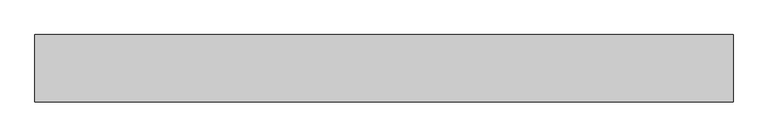
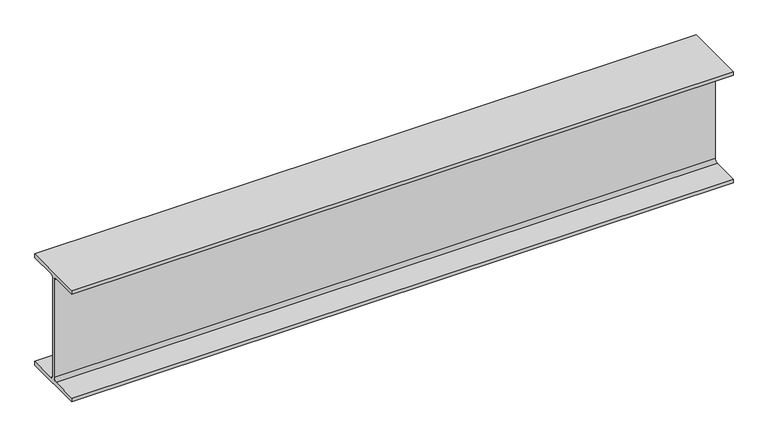
"""IFC4 building model written with IfcOpenShell, lengths in millimetres: beam geometry, Old_Steel Beam_H-KSD3502 : H_SB_ASB_H-200×200x8x12."""

from ifc_helpers import new_model, si_unit, point, frame, frame_2d, origin, place, context, project, spatial, polyline, circle_curve, trimmed, segment, composite_curve, outline, extrude, source, transform, mapped, element, save


def beam_c4b8d585(model_context):
    return source(origin(), model_context, "Body", "SweptSolid", [
        extrude(outline(composite_curve([segment(polyline([(82.5, -141.5), (82.5, -151.7), (-82.5, -151.7), (-82.5, -141.5), (-11.9, -141.5)]), True, "CONTINUOUS"), segment(trimmed(circle_curve(frame_2d((-11.9, -132.6)), 8.9), [point((-11.9, -141.5))], [point((-3.0, -132.6))], True, "CARTESIAN"), True, "CONTINUOUS"), segment(polyline([(-3.0, -132.6), (-3.0, 132.6)]), True, "CONTINUOUS"), segment(trimmed(circle_curve(frame_2d((-11.9, 132.6)), 8.9), [point((-3.0, 132.6))], [point((-11.9, 141.5))], True, "CARTESIAN"), True, "CONTINUOUS"), segment(polyline([(-11.9, 141.5), (-82.5, 141.5), (-82.5, 151.7), (82.5, 151.7), (82.5, 141.5), (11.9, 141.5)]), True, "CONTINUOUS"), segment(trimmed(circle_curve(frame_2d((11.9, 132.6)), 8.9), [point((11.9, 141.5))], [point((3.0, 132.6))], True, "CARTESIAN"), True, "CONTINUOUS"), segment(polyline([(3.0, 132.6), (3.0, -132.6)]), True, "CONTINUOUS"), segment(trimmed(circle_curve(frame_2d((11.9, -132.6)), 8.9), [point((3.0, -132.6))], [point((11.9, -141.5))], True, "CARTESIAN"), True, "CONTINUOUS"), segment(polyline([(11.9, -141.5), (82.5, -141.5)]), True, "CONTINUOUS")], self_intersect=False)), frame((-969.5119577, 0.0, 0.0), z_axis=(1.0, 0.0, 0.0), x_axis=(0.0, 1.0, 0.0)), (0.0, 0.0, 1.0), 1706.6963833),
    ])


if __name__ == "__main__":
    model = new_model("IFC4")
    model_context = context("Model", 3, world=origin())
    ifc_project = project(units=[si_unit("LENGTHUNIT", "METRE", prefix="MILLI")], contexts=[model_context])
    site = spatial("IfcSite", under=ifc_project)
    building = spatial("IfcBuilding", under=site)
    placement = place(None, origin())
    beam_shape = beam_c4b8d585(model_context)
    element("IfcBeam", 1, ObjectType="Old_Steel Beam_H-KSD3502 : H_SB_ASB_H-200×200x8x12", at=placement, inside=building, context=model_context, shape_type="MappedRepresentation", body=[
        mapped(beam_shape, transform((0.0, 0.0, 0.0), x_axis=(1.0, 0.0, 0.0), y_axis=(0.0, 1.0, 0.0), z_axis=(0.0, 0.0, 1.0))),
    ])
    save(model, "model.ifc")

# Revit data of these elements
# Type "Old_Steel Beam_H-KSD3502 : H_SB_ASB_H-200×200x8x12"
#   Width = 20.0 cm
#   Web Thickness = 0.8 cm
#   Web Fillet = 1.3 cm
#   Warping Constant = 141376.0 cm⁶
#   Torsional Moment of Inertia = 26.2485 cm⁴
#   Torsional Modulus = 1.0 cm³
#   Section Area = 63.53 cm²
#   Plastic Modulus weak axis = 244.0 cm³
#   Plastic Modulus strong axis = 525.0 cm³
#   Perimeter = 1.16 m²/m
#   Nominal Weight = 49.90 kgf/m
#   Moment of Inertia weak axis = 1600.00 cm⁴
#   Moment of Inertia strong axis = 4720.00 cm⁴
#   Height = 20.0 cm
#   Flange Thickness = 1.2 cm
#   Elastic Modulus weak axis = 160.0 cm³
#   Elastic Modulus strong axis = 472.0 cm³
#   Centroid Vertical = 10.0 cm
#   Centroid Horizontal = 10.0 cm
#   Length [instance default] = 1.5240 m
#   Structural Material [instance default] = Steel, 45-345
#   Assembly Code = ""
# Element 1 (IfcBeam, "Old_Steel Beam_H-KSD3502 : H_SB_ASB_H-200×200x8x12")
#   Structural Material = none
# Materials
#   "Steel, 45-345": class "Metal", colour RGB 189 187 185, transparency 0, Description = "Steel 345 MPa", Cost = 0
